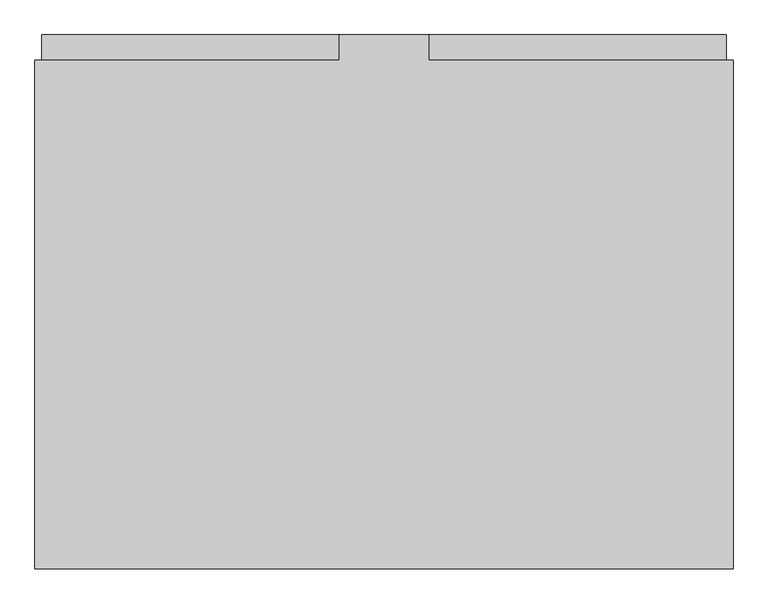
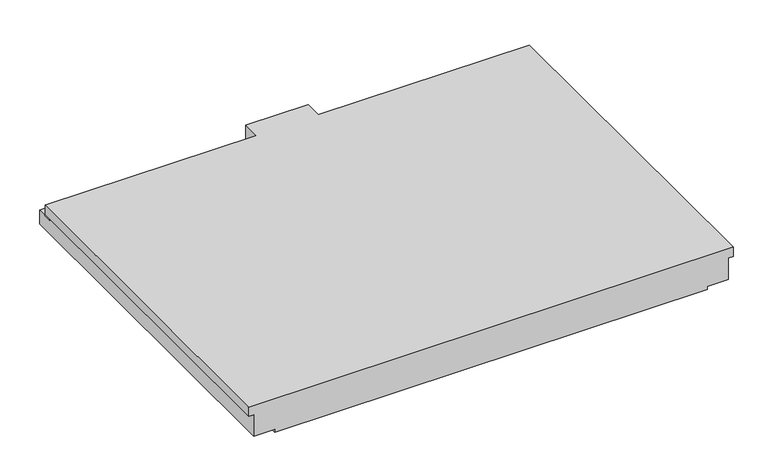
"""IFC4 building model written with IfcOpenShell, lengths in millimetres: proxy geometry, NLRS_24_GM_UN_rechthoekig bordes prefab-AV_gen_rsf : prefab bordes_gen__2300x3005."""

from ifc_helpers import new_model, si_unit, origin, place, context, project, spatial, faceted_brep, source, transform, mapped, element, save


def generic_models_f0e5f7b1(model_context):
    return source(origin(), model_context, "Body", "Brep", [
        faceted_brep([(1502.5, 2190.0, 0.0), (1502.5, 0.0, 0.0), (1502.5, 0.0, -60.0), (1502.5, 2190.0, -60.0), (192.5, 2300.0, -110.0), (192.5, 2190.0, -110.0), (1472.5, 2190.0, -110.0), (1472.5, 2300.0, -110.0), (192.5, 2190.0, 0.0), (1472.5, 2190.0, -60.0), (192.5, 2300.0, 0.0), (-192.5, 2300.0, 0.0), (-192.5, 2300.0, -110.0), (-192.5, 2190.0, -110.0), (-192.5, 2190.0, 0.0), (-1502.5, 0.0, 0.0), (-1502.5, 2190.0, 0.0), (-1502.5, 2190.0, -60.0), (-1502.5, 0.0, -60.0), (-1472.5, 2300.0, -110.0), (1472.5, 2300.0, -200.0), (1342.5, 2300.0, -200.0), (1342.5, 2300.0, -220.0), (-1342.5, 2300.0, -220.0), (-1342.5, 2300.0, -200.0), (-1472.5, 2300.0, -200.0), (-1472.5, 2190.0, -110.0), (-1472.5, 2190.0, -60.0), (-1472.5, 0.0, -60.0), (-1472.5, 0.0, -200.0), (-1342.5, 0.0, -200.0), (-1342.5, 0.0, -220.0), (1342.5, 0.0, -220.0), (1342.5, 0.0, -200.0), (1472.5, 0.0, -200.0), (1472.5, 0.0, -60.0)], [[[0, 1, 2, 3]], [[4, 5, 6, 7]], [[8, 0, 3, 9, 6, 5]], [[10, 8, 5, 4]], [[11, 12, 13, 14]], [[15, 16, 17, 18]], [[19, 12, 11, 10, 4, 7, 20, 21, 22, 23, 24, 25]], [[12, 19, 26, 13]], [[16, 14, 13, 26, 27, 17]], [[16, 15, 1, 0, 8, 10, 11, 14]], [[15, 18, 28, 29, 30, 31, 32, 33, 34, 35, 2, 1]], [[31, 23, 22, 32]], [[27, 28, 18, 17]], [[25, 29, 28, 27, 26, 19]], [[29, 25, 24, 30]], [[30, 24, 23, 31]], [[35, 9, 3, 2]], [[34, 20, 7, 6, 9, 35]], [[20, 34, 33, 21]], [[21, 33, 32, 22]]]),
    ])


if __name__ == "__main__":
    model = new_model("IFC4")
    model_context = context("Model", 3, world=origin())
    ifc_project = project(units=[si_unit("LENGTHUNIT", "METRE", prefix="MILLI")], contexts=[model_context])
    site = spatial("IfcSite", under=ifc_project)
    building = spatial("IfcBuilding", under=site)
    placement = place(None, origin())
    generic_models_shape = generic_models_f0e5f7b1(model_context)
    element("IfcBuildingElementProxy", 1, Name="NLRS_24_GM_UN_rechthoekig bordes prefab-AV_gen_rsf : prefab bordes_gen__2300x3005", ObjectType="NLRS_24_GM_UN_rechthoekig bordes prefab-AV_gen_rsf : prefab bordes_gen__2300x3005", at=placement, inside=building, context=model_context, shape_type="MappedRepresentation", body=[
        mapped(generic_models_shape, transform((0.0, 0.0, 0.0), x_axis=(1.0, 0.0, 0.0), y_axis=(0.0, 1.0, 0.0), z_axis=(0.0, 0.0, 1.0))),
    ])
    save(model, "model.ifc")

# Revit data of these elements
# Type "NLRS_24_GM_UN_rechthoekig bordes prefab-AV_gen_rsf : prefab bordes_gen__2300x3005"
#   Export Type to IFC As = "IfcStair"
#   Type IfcGUID = "2CEqVLPNH8KRN7ghwV3abv"
#   Type Comments = " "
#   Model = " "
#   Manufacturer = " "
#   Description = "rechthoekig bordes prefab\r\n1930x4395"
#   Assembly Code = "24.15"
#   Width = 3005 mm
#   Thickness = 220 mm
#   Perimeter = 10610 mm
#   NLRS_C_lengte_02 = 1310 mm
#   NLRS_C_lengte_01 = 1310 mm
#   NLRS_C_hoogte_02 = 110 mm
#   NLRS_C_hoogte_01 = 110 mm
#   NLRS_C_diepte_04 = 2300 mm
#   NLRS_C_diepte_03 = 2300 mm
#   NLRS_C_diepte_02 = 110 mm
#   NLRS_C_diepte_01 = 110 mm
#   Length = 2300 mm
#   Default Elevation = 1219.2 mm
#   Area = 6.9115 m²
#   NLRS_C_materiaal = NLRS_f2_beton prefab_gen_rsf
#   Keynote = ""
# Element 1 (IfcBuildingElementProxy, "NLRS_24_GM_UN_rechthoekig bordes prefab-AV_gen_rsf : prefab bordes_gen__2300x3005")
#   Materials on its faces: "NLRS_f2_beton prefab_gen_rsf"
# Materials
#   "NLRS_f2_beton prefab_gen_rsf": class "F - Niet gebakken kunststeen", colour RGB 129 133 118, transparency 0, Keynote = "f2", Manufacturer = "Revit Standards Foundation", URL = "www.revitstandards.org", Description = "beton prefab", Cost = 0
